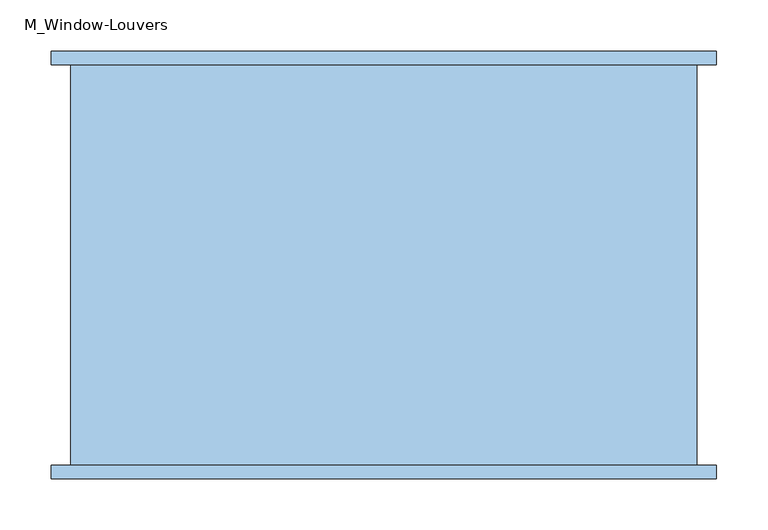
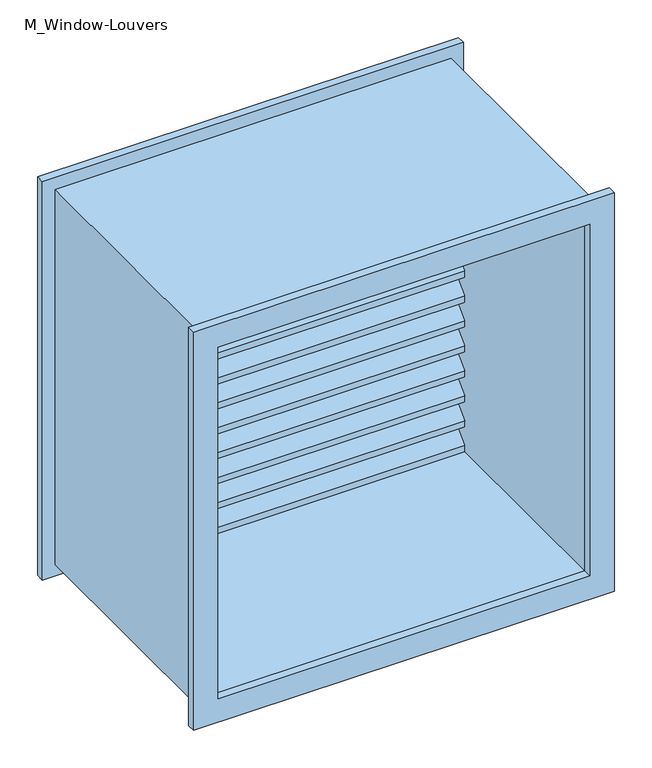
"""IFC4 building model written with IfcOpenShell, lengths in millimetres: window geometry, M_Window-Louvers : H_WD_AMW_AL Louver_W610xH610."""

import ifcopenshell
import ifcopenshell.guid

model = None  # the IFC model being written
_history = None  # IfcOwnerHistory: only IFC2X3 demands one
_inside = {}  # id of a spatial element -> (the spatial element, [elements in it])
_under = {}  # id of a project, library or spatial element -> (it, [spatial elements below it])
_declared = {}  # id of a project -> (the project, [libraries it declares])
_typed = {}  # id of a type object -> (the type object, [elements of that type])
_made_of = {}  # id of a material, layer set ... -> (it, [elements and type objects made of it])


def new_model(schema):
    """Start an empty IFC model of exactly this schema.

    Asked for "IFC4X3", IfcOpenShell would pick the latest addendum, in which some entities
    have other attributes; the version numbers below select the first issue.
    IFC2X3 requires an IfcOwnerHistory on every rooted entity: one is made here for all.
    """
    global model, _history
    if schema == "IFC4X3":
        model = ifcopenshell.file(schema_version=(4, 3, 0, 0))
    else:
        model = ifcopenshell.file(schema=schema)
    _inside.clear()
    _under.clear()
    _declared.clear()
    _typed.clear()
    _made_of.clear()
    _history = None
    if model.schema == "IFC2X3":
        org = make("IfcOrganization", Name="unknown")
        user = make(
            "IfcPersonAndOrganization",
            ThePerson=make("IfcPerson", FamilyName="unknown"),
            TheOrganization=org,
        )
        app = make(
            "IfcApplication",
            ApplicationDeveloper=org,
            Version="unknown",
            ApplicationFullName="unknown",
            ApplicationIdentifier="unknown",
        )
        _history = make(
            "IfcOwnerHistory",
            OwningUser=user,
            OwningApplication=app,
            ChangeAction="ADDED",
            CreationDate=0,
        )
    return model


def make(cls, **values):
    """One entity of the class cls with the attributes given. An attribute that is None is left unset."""
    return model.create_entity(
        cls, **{name: value for name, value in values.items() if value is not None}
    )


def rooted(cls, **values):
    """An entity with a GlobalId (a new one), such as an element, a storey or a relation."""
    return make(cls, GlobalId=ifcopenshell.guid.new(), OwnerHistory=_history, **values)


def si_unit(unit_type, name, prefix=None):
    """IfcSIUnit, for example si_unit("LENGTHUNIT", "METRE", prefix="MILLI")."""
    return make("IfcSIUnit", UnitType=unit_type, Prefix=prefix, Name=name)


def assignment(units):
    """IfcUnitAssignment: the units of a project."""
    return None if units is None else make("IfcUnitAssignment", Units=units)


def point(xyz):
    """IfcCartesianPoint."""
    return None if xyz is None else make("IfcCartesianPoint", Coordinates=xyz)


def direction(xyz):
    """IfcDirection."""
    return None if xyz is None else make("IfcDirection", DirectionRatios=xyz)


def frame(location, z_axis=None, x_axis=None):
    """IfcAxis2Placement3D, a coordinate frame: its origin and axes. An axis left out is left unset."""
    return make(
        "IfcAxis2Placement3D",
        Location=point(location),
        Axis=direction(z_axis),
        RefDirection=direction(x_axis),
    )


def origin():
    """The frame at (0, 0, 0) with its axes left unset."""
    return frame((0.0, 0.0, 0.0))


def place(relative_to, where):
    """IfcLocalPlacement: puts the frame where relative to a parent placement (None: the world)."""
    return make(
        "IfcLocalPlacement", PlacementRelTo=relative_to, RelativePlacement=where
    )


def context(
    kind, dimensions, precision=None, world=None, true_north=None, identifier=None
):
    """IfcGeometricRepresentationContext, for example the 3D "Model" context."""
    return make(
        "IfcGeometricRepresentationContext",
        ContextIdentifier=identifier,
        ContextType=kind,
        CoordinateSpaceDimension=dimensions,
        Precision=precision,
        WorldCoordinateSystem=world,
        TrueNorth=true_north,
    )


def project(units=None, contexts=None):
    """IfcProject with its units and contexts."""
    return rooted(
        "IfcProject",
        Name="project",
        RepresentationContexts=contexts,
        UnitsInContext=assignment(units),
    )


def spatial(cls, under=None, at=None, **own):
    """A site, building, storey or space (cls), placed at a placement, below another one or the project."""
    s = rooted(cls, ObjectPlacement=at, **own)
    if under is not None:
        _under.setdefault(under.id(), (under, []))[1].append(s)
    return s


def polyline(points):
    """IfcPolyline through the points."""
    return make("IfcPolyline", Points=[point(p) for p in points])


def outline(outer, holes=None, kind="AREA"):
    """IfcArbitraryClosedProfileDef: a profile drawn as a closed curve; with holes, ...WithVoids."""
    if holes is None:
        return make("IfcArbitraryClosedProfileDef", ProfileType=kind, OuterCurve=outer)
    return make(
        "IfcArbitraryProfileDefWithVoids",
        ProfileType=kind,
        OuterCurve=outer,
        InnerCurves=holes,
    )


def extrude(swept, where, along, depth):
    """IfcExtrudedAreaSolid: the profile swept, set in the frame where, extruded along a direction by depth."""
    return make(
        "IfcExtrudedAreaSolid",
        SweptArea=swept,
        Position=where,
        ExtrudedDirection=direction(along),
        Depth=depth,
    )


def shape(context_of_items, identifier, shape_type, items):
    """IfcShapeRepresentation: the items that make up one representation, for example the "Body"."""
    return make(
        "IfcShapeRepresentation",
        ContextOfItems=context_of_items,
        RepresentationIdentifier=identifier,
        RepresentationType=shape_type,
        Items=items,
    )


def source(mapping_origin, context_of_items, identifier, shape_type, items):
    """IfcRepresentationMap: a shape defined once, which mapped items show again and again."""
    return make(
        "IfcRepresentationMap",
        MappingOrigin=mapping_origin,
        MappedRepresentation=shape(context_of_items, identifier, shape_type, items),
    )


def transform(
    local_origin,
    x_axis=None,
    y_axis=None,
    z_axis=None,
    scale=None,
    scale2=None,
    scale3=None,
    uniform=True,
):
    """IfcCartesianTransformationOperator3D, or its non-uniform kind. x_axis, y_axis, z_axis: its Axis1, 2, 3."""
    if uniform:
        return make(
            "IfcCartesianTransformationOperator3D",
            Axis1=direction(x_axis),
            Axis2=direction(y_axis),
            LocalOrigin=point(local_origin),
            Scale=scale,
            Axis3=direction(z_axis),
        )
    return make(
        "IfcCartesianTransformationOperator3DnonUniform",
        Axis1=direction(x_axis),
        Axis2=direction(y_axis),
        LocalOrigin=point(local_origin),
        Scale=scale,
        Axis3=direction(z_axis),
        Scale2=scale2,
        Scale3=scale3,
    )


def mapped(mapping_source, mapping_target):
    """IfcMappedItem: shows the shape of a source again, moved by a transform."""
    return make(
        "IfcMappedItem", MappingSource=mapping_source, MappingTarget=mapping_target
    )


def made_of(thing, what):
    """Note that an element or type object is made of a material, layer set ...; save() writes the relation."""
    if what is not None:
        _made_of.setdefault(what.id(), (what, []))[1].append(thing)
    return thing


def element(
    cls,
    number,
    at=None,
    inside=None,
    cuts=None,
    type_object=None,
    material=None,
    context=None,
    identifier="Body",
    shape_type=None,
    held_by="IfcProductDefinitionShape",
    body=None,
    shapes=None,
    **own,
):
    """One element of the class cls, such as IfcWall. Its Tag is "e" and its number.

    at: its placement. inside: the storey or other place that contains it. cuts: it is an
    opening in that element (IfcRelVoidsElement). A single representation is given by context,
    identifier, shape_type and body (its items); several are given by shapes. held_by: the class
    of the entity that holds the representations. save() writes the other relations.
    """
    e = rooted(cls, Tag="e%d" % number, ObjectPlacement=at, **own)
    if body is not None:
        shapes = [shape(context, identifier, shape_type, body)]
    if shapes is not None:
        e.Representation = make(held_by, Representations=shapes)
    if inside is not None:
        _inside.setdefault(inside.id(), (inside, []))[1].append(e)
    if cuts is not None:
        rooted(
            "IfcRelVoidsElement", RelatingBuildingElement=cuts, RelatedOpeningElement=e
        )
    if type_object is not None:
        _typed.setdefault(type_object.id(), (type_object, []))[1].append(e)
    return made_of(e, material)


def aggregate(whole, parts):
    """IfcRelAggregates: a whole, such as a stair, and the parts it consists of."""
    return rooted("IfcRelAggregates", RelatingObject=whole, RelatedObjects=parts)


def save(model, path):
    """Write the relations noted so far, then the file.

    IfcRelAggregates (storeys below a building ...), IfcRelContainedInSpatialStructure (elements
    in a storey), IfcRelDefinesByType, IfcRelAssociatesMaterial and IfcRelDeclares: one each for
    every whole, place, type object, material and project.
    """
    for whole, parts in _under.values():
        aggregate(whole, parts)
    for where, things in _inside.values():
        rooted(
            "IfcRelContainedInSpatialStructure",
            RelatedElements=things,
            RelatingStructure=where,
        )
    for kind, things in _typed.values():
        rooted("IfcRelDefinesByType", RelatedObjects=things, RelatingType=kind)
    for what, things in _made_of.values():
        rooted("IfcRelAssociatesMaterial", RelatedObjects=things, RelatingMaterial=what)
    for by, libraries in _declared.values():
        rooted("IfcRelDeclares", RelatingContext=by, RelatedDefinitions=libraries)
    model.write(path)


def m_window_louvers_33c5b602(model_context):
    return source(origin(), model_context, "Body", "SweptSolid", [
        extrude(outline(polyline([(188.65, 1430.5146859), (188.65, 1420.4737696), (153.725, 1455.3987696), (118.8, 1420.4737696), (118.8, 1430.5146859), (153.725, 1465.4396859), (188.65, 1430.5146859)])), frame((-286.0, 0.0, 0.0), z_axis=(1.0, 0.0, 0.0), x_axis=(0.0, 1.0, 0.0)), (0.0, 0.0, 1.0), 572.0),
        extrude(outline(polyline([(188.65, 1389.9793717), (188.65, 1379.9384554), (153.725, 1414.8634554), (118.8, 1379.9384554), (118.8, 1389.9793717), (153.725, 1424.9043717), (188.65, 1389.9793717)])), frame((-286.0, 0.0, 0.0), z_axis=(1.0, 0.0, 0.0), x_axis=(0.0, 1.0, 0.0)), (0.0, 0.0, 1.0), 572.0),
        extrude(outline(polyline([(188.65, 1349.4440576), (188.65, 1339.4031413), (153.725, 1374.3281413), (118.8, 1339.4031413), (118.8, 1349.4440576), (153.725, 1384.3690576), (188.65, 1349.4440576)])), frame((-286.0, 0.0, 0.0), z_axis=(1.0, 0.0, 0.0), x_axis=(0.0, 1.0, 0.0)), (0.0, 0.0, 1.0), 572.0),
        extrude(outline(polyline([(188.65, 1308.9087435), (188.65, 1298.8678272), (153.725, 1333.7928272), (118.8, 1298.8678272), (118.8, 1308.9087435), (153.725, 1343.8337435), (188.65, 1308.9087435)])), frame((-286.0, 0.0, 0.0), z_axis=(1.0, 0.0, 0.0), x_axis=(0.0, 1.0, 0.0)), (0.0, 0.0, 1.0), 572.0),
        extrude(outline(polyline([(188.65, 1268.3734293), (188.65, 1258.3325131), (153.725, 1293.2575131), (118.8, 1258.3325131), (118.8, 1268.3734293), (153.725, 1303.2984293), (188.65, 1268.3734293)])), frame((-286.0, 0.0, 0.0), z_axis=(1.0, 0.0, 0.0), x_axis=(0.0, 1.0, 0.0)), (0.0, 0.0, 1.0), 572.0),
        extrude(outline(polyline([(188.65, 1227.8381152), (188.65, 1217.7971989), (153.725, 1252.7221989), (118.8, 1217.7971989), (118.8, 1227.8381152), (153.725, 1262.7631152), (188.65, 1227.8381152)])), frame((-286.0, 0.0, 0.0), z_axis=(1.0, 0.0, 0.0), x_axis=(0.0, 1.0, 0.0)), (0.0, 0.0, 1.0), 572.0),
        extrude(outline(polyline([(188.65, 1187.3028011), (188.65, 1177.2618848), (153.725, 1212.1868848), (118.8, 1177.2618848), (118.8, 1187.3028011), (153.725, 1222.2278011), (188.65, 1187.3028011)])), frame((-286.0, 0.0, 0.0), z_axis=(1.0, 0.0, 0.0), x_axis=(0.0, 1.0, 0.0)), (0.0, 0.0, 1.0), 572.0),
        extrude(outline(polyline([(188.65, 1146.7674869), (188.65, 1136.7265707), (153.725, 1171.6515707), (118.8, 1136.7265707), (118.8, 1146.7674869), (153.725, 1181.6924869), (188.65, 1146.7674869)])), frame((-286.0, 0.0, 0.0), z_axis=(1.0, 0.0, 0.0), x_axis=(0.0, 1.0, 0.0)), (0.0, 0.0, 1.0), 572.0),
        extrude(outline(polyline([(188.65, 1106.2321728), (188.65, 1096.1912565), (153.725, 1131.1162565), (118.8, 1096.1912565), (118.8, 1106.2321728), (153.725, 1141.1571728), (188.65, 1106.2321728)])), frame((-286.0, 0.0, 0.0), z_axis=(1.0, 0.0, 0.0), x_axis=(0.0, 1.0, 0.0)), (0.0, 0.0, 1.0), 572.0),
        extrude(outline(polyline([(188.65, 1065.6968587), (188.65, 1055.6559424), (153.725, 1090.5809424), (118.8, 1055.6559424), (118.8, 1065.6968587), (153.725, 1100.6218587), (188.65, 1065.6968587)])), frame((-286.0, 0.0, 0.0), z_axis=(1.0, 0.0, 0.0), x_axis=(0.0, 1.0, 0.0)), (0.0, 0.0, 1.0), 572.0),
        extrude(outline(polyline([(188.65, 1025.1615446), (188.65, 1015.1206283), (153.725, 1050.0456283), (118.8, 1015.1206283), (118.8, 1025.1615446), (153.725, 1060.0865446), (188.65, 1025.1615446)])), frame((-286.0, 0.0, 0.0), z_axis=(1.0, 0.0, 0.0), x_axis=(0.0, 1.0, 0.0)), (0.0, 0.0, 1.0), 572.0),
        extrude(outline(polyline([(188.65, 984.6262304), (188.65, 974.5853141), (153.725, 1009.5103141), (118.8, 974.5853141), (118.8, 984.6262304), (153.725, 1019.5512304), (188.65, 984.6262304)])), frame((-286.0, 0.0, 0.0), z_axis=(1.0, 0.0, 0.0), x_axis=(0.0, 1.0, 0.0)), (0.0, 0.0, 1.0), 572.0),
        extrude(outline(polyline([(188.65, 1471.05), (188.65, 1461.0090837), (153.725, 1495.9340837), (118.8, 1461.0090837), (118.8, 1471.05), (153.725, 1505.975), (188.65, 1471.05)])), frame((-286.0, 0.0, 0.0), z_axis=(1.0, 0.0, 0.0), x_axis=(0.0, 1.0, 0.0)), (0.0, 0.0, 1.0), 572.0),
        extrude(outline(polyline([(188.65, 944.0909163), (188.65, 934.05), (153.725, 968.975), (118.8, 934.05), (118.8, 944.0909163), (153.725, 979.0159163), (188.65, 944.0909163)])), frame((-286.0, 0.0, 0.0), z_axis=(1.0, 0.0, 0.0), x_axis=(0.0, 1.0, 0.0)), (0.0, 0.0, 1.0), 572.0),
        extrude(outline(polyline([(1543.975, -323.95), (896.05, -323.95), (896.05, 323.95), (1543.975, 323.95), (1543.975, -323.95)]), holes=[polyline([(1505.95, -285.95), (1505.95, 285.95), (934.05, 285.95), (934.05, -285.95), (1505.95, -285.95)])]), frame((0.0, 188.65, 0.0), z_axis=(0.0, 1.0, 0.0), x_axis=(0.0, 0.0, 1.0)), (0.0, 0.0, 1.0), 13.0),
        extrude(outline(polyline([(1543.975, 323.95), (1543.975, -323.95), (896.05, -323.95), (896.05, 323.95), (1543.975, 323.95)]), holes=[polyline([(1505.975, 285.95), (934.05, 285.95), (934.05, -285.95), (1505.975, -285.95), (1505.975, 285.95)])]), frame((0.0, -214.35, 0.0), z_axis=(0.0, 1.0, 0.0), x_axis=(0.0, 0.0, 1.0)), (0.0, 0.0, 1.0), 13.0),
        extrude(outline(polyline([(1525.0, 305.0), (1525.0, -305.0), (915.0, -305.0), (915.0, 305.0), (1525.0, 305.0)]), holes=[polyline([(1505.95, 285.95), (934.05, 285.95), (934.05, -285.95), (1505.95, -285.95), (1505.95, 285.95)])]), frame((0.0, -201.35, 0.0), z_axis=(0.0, 1.0, 0.0), x_axis=(0.0, 0.0, 1.0)), (0.0, 0.0, 1.0), 390.0),
    ])


if __name__ == "__main__":
    model = new_model("IFC4")
    model_context = context("Model", 3, world=origin())
    ifc_project = project(units=[si_unit("LENGTHUNIT", "METRE", prefix="MILLI")], contexts=[model_context])
    site = spatial("IfcSite", under=ifc_project)
    building = spatial("IfcBuilding", under=site)
    placement = place(None, origin())
    m_window_louvers_shape = m_window_louvers_33c5b602(model_context)
    element("IfcWindow", 1, ObjectType="M_Window-Louvers : H_WD_AMW_AL Louver_W610xH610", at=placement, inside=building, context=model_context, shape_type="MappedRepresentation", body=[
        mapped(m_window_louvers_shape, transform((0.0, 0.0, 0.0), x_axis=(1.0, 0.0, 0.0), y_axis=(0.0, 1.0, 0.0), z_axis=(0.0, 0.0, 1.0))),
    ])
    save(model, "model.ifc")

# Revit data of these elements
# Project information
#   Building Name = "MAIN GATE SECURITY BUILDING"
#   Project Status = "Project Status"
#   Client Name = "현대엔지니어링"
#   Project Address = "서울시 종로구 율곡로 75(계동)"
#   Project Name = "Therma Visayas Energy Project"
#   Project Number = "-"
#   BuildingbookInternationalBuildNumber = "ZgA=BAAAAA==2023BgFlAAAAAQoAAAABAQAAAAYBZAAAAAHnBwAABAQAAAABWwIAAAcH0"
# Type "M_Window-Louvers : H_WD_AMW_AL Louver_W610xH610"
#   Type Mark = "AL"
#   Construction Type Id = "GSP4R"
#   Analytic Construction = "1/8 in Pilkington single glazing"
#   Visual Light Transmittance = 0.9
#   Thermal Resistance (R) = 0.271106 (m²·K)/W
#   Solar Heat Gain Coefficient = 0.78
#   Max Height = 0.603598 m
#   Height = 0.6100 m
#   Heat Transfer Coefficient (U) = 3.6886 W/(m²·K)
#   Default Sill Height = 0.9150 m
#   Trim Projection_Exterior = 0.0130 m
#   Trim Projection_Interior = 0.0130 m
#   Trim Width_Exterior = 0.0380 m
#   Trim Width_Interior = 0.0380 m
#   Width = 0.6100 m
#   Blade Width = 0.5720 m
#   Blade Vertical Thickness = 0.010041 m
#   Blade Thickness = 0.0071 m
#   Blade Spacing = 0.0300 m
#   Blade Height = 0.044966 m
#   Blade Depth = 0.06985 m
#   Blade Angle = 45.00°
#   Max Blade Count = 14
#   Define Thermal Properties by = 1
#   Blade Count = 14
#   Frame Material = Birch
#   Louvers Material = Birch
#   Trim Exterior Material = Birch
#   Trim Interior Material = Birch
#   Wall Closure = (empty or 0)
# Element 1 (IfcWindow, "M_Window-Louvers : H_WD_AMW_AL Louver_W610xH610")
#   Materials on its faces: "Birch"
# Materials
#   "Birch": class "Wood", colour RGB 224 178 126, transparency 0, Description = "Betula Alleghaniensis", Cost = 0
